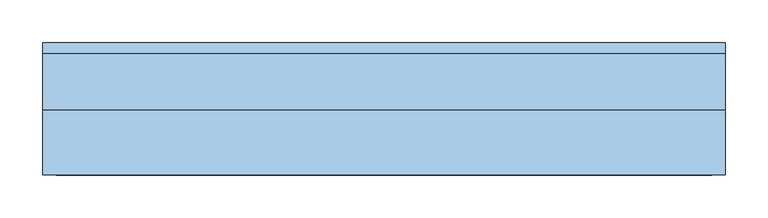
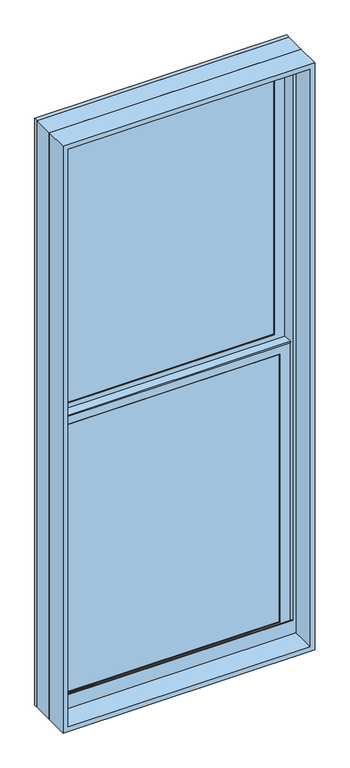
"""IFC4 building model written with IfcOpenShell, lengths in millimetres: window geometry, Window-Double_Hung-Marvin-Essential : ESDH2866."""

from ifc_helpers import new_model, si_unit, frame, origin, place, context, project, spatial, polyline, outline, extrude, faceted_brep, source, transform, mapped, element, save


def window_37e84bf3(model_context):
    return source(origin(), model_context, "Body", "SolidModel", [
        extrude(outline(polyline([(123.825, 20.6375), (123.825, 15.875), (104.775, 15.875), (104.775, 20.6375), (123.825, 20.6375)])), frame((0.0, 0.0, 527.05), z_axis=(0.0, 0.0, 1.0), x_axis=(1.0, 0.0, 0.0)), (0.0, 0.0, 1.0), 908.05),
        extrude(outline(polyline([(-104.775, 20.6375), (-104.775, 15.875), (-123.825, 15.875), (-123.825, 20.6375), (-104.775, 20.6375)])), frame((0.0, 0.0, 527.05), z_axis=(0.0, 0.0, 1.0), x_axis=(1.0, 0.0, 0.0)), (0.0, 0.0, 1.0), 908.05),
        extrude(outline(polyline([(342.9, 20.6375), (342.9, 15.875), (-342.9, 15.875), (-342.9, 20.6375), (342.9, 20.6375)])), frame((0.0, 0.0, 971.55), z_axis=(0.0, 0.0, 1.0), x_axis=(1.0, 0.0, 0.0)), (0.0, 0.0, 1.0), 19.05),
        extrude(outline(polyline([(-123.825, 46.83125), (-123.825, 51.59375), (-104.775, 51.59375), (-104.775, 46.83125), (-123.825, 46.83125)])), frame((0.0, 0.0, 1473.2), z_axis=(0.0, 0.0, 1.0), x_axis=(1.0, 0.0, 0.0)), (0.0, 0.0, 1.0), 908.05),
        extrude(outline(polyline([(104.775, 46.83125), (104.775, 51.59375), (123.825, 51.59375), (123.825, 46.83125), (104.775, 46.83125)])), frame((0.0, 0.0, 1473.2), z_axis=(0.0, 0.0, 1.0), x_axis=(1.0, 0.0, 0.0)), (0.0, 0.0, 1.0), 908.05),
        extrude(outline(polyline([(-342.9, 46.83125), (-342.9, 51.59375), (342.9, 51.59375), (342.9, 46.83125), (-342.9, 46.83125)])), frame((0.0, 0.0, 1917.7), z_axis=(0.0, 0.0, 1.0), x_axis=(1.0, 0.0, 0.0)), (0.0, 0.0, 1.0), 19.05),
        extrude(outline(polyline([(123.825, 20.6375), (104.775, 20.6375), (104.775, 25.4), (123.825, 25.4), (123.825, 20.6375)])), frame((0.0, 0.0, 527.05), z_axis=(0.0, 0.0, 1.0), x_axis=(1.0, 0.0, 0.0)), (0.0, 0.0, 1.0), 908.05),
        extrude(outline(polyline([(-104.775, 20.6375), (-123.825, 20.6375), (-123.825, 25.4), (-104.775, 25.4), (-104.775, 20.6375)])), frame((0.0, 0.0, 527.05), z_axis=(0.0, 0.0, 1.0), x_axis=(1.0, 0.0, 0.0)), (0.0, 0.0, 1.0), 908.05),
        extrude(outline(polyline([(342.9, 20.6375), (-342.9, 20.6375), (-342.9, 25.4), (342.9, 25.4), (342.9, 20.6375)])), frame((0.0, 0.0, 971.55), z_axis=(0.0, 0.0, 1.0), x_axis=(1.0, 0.0, 0.0)), (0.0, 0.0, 1.0), 19.05),
        extrude(outline(polyline([(-123.825, 56.35625), (-104.775, 56.35625), (-104.775, 51.59375), (-123.825, 51.59375), (-123.825, 56.35625)])), frame((0.0, 0.0, 1473.2), z_axis=(0.0, 0.0, 1.0), x_axis=(1.0, 0.0, 0.0)), (0.0, 0.0, 1.0), 908.05),
        extrude(outline(polyline([(104.775, 56.35625), (123.825, 56.35625), (123.825, 51.59375), (104.775, 51.59375), (104.775, 56.35625)])), frame((0.0, 0.0, 1473.2), z_axis=(0.0, 0.0, 1.0), x_axis=(1.0, 0.0, 0.0)), (0.0, 0.0, 1.0), 908.05),
        extrude(outline(polyline([(-342.9, 56.35625), (342.9, 56.35625), (342.9, 51.59375), (-342.9, 51.59375), (-342.9, 56.35625)])), frame((0.0, 0.0, 1917.7), z_axis=(0.0, 0.0, 1.0), x_axis=(1.0, 0.0, 0.0)), (0.0, 0.0, 1.0), 19.05),
        faceted_brep([(-369.8875, 5.6780605, 1465.1351748), (-369.8875, 5.6780605, 1460.5), (369.8875, 5.6780605, 1460.5), (369.8875, 5.6780605, 1465.1351748), (-369.8875, 34.8118605, 1465.1351748), (369.8875, 34.8118605, 1465.1351748), (369.8875, 34.8118605, 1460.5), (-369.8875, 34.8118605, 1460.5), (-369.8875, 30.1625, 1460.5), (-369.8875, 30.1625, 500.0625), (-369.8875, 8.9241104, 500.0625), (-369.8875, 8.9241104, 1460.5), (369.8875, 8.9241104, 1460.5), (369.8875, 30.1625, 1460.5), (369.8875, 8.9241104, 500.0625), (369.8875, 30.1625, 500.0625), (-354.0034752, 11.90625, 1446.2034752), (-354.0034752, 30.1625, 1446.2034752), (354.0034752, 30.1625, 1446.2034752), (354.0034752, 11.90625, 1446.2034752), (-337.34375, 10.4662439, 1429.54375), (-337.34375, 11.90625, 1429.54375), (337.34375, 11.90625, 1429.54375), (337.34375, 10.4662439, 1429.54375), (338.8858834, 8.9241104, 1431.0858834), (-338.8858834, 8.9241104, 1431.0858834), (354.0034752, 30.1625, 515.9465248), (354.0034752, 11.90625, 515.9465248), (337.34375, 11.90625, 532.60625), (337.34375, 10.4662439, 532.60625), (338.8858834, 8.9241104, 531.0641166), (-354.0034752, 30.1625, 515.9465248), (-354.0034752, 11.90625, 515.9465248), (-337.34375, 11.90625, 532.60625), (-337.34375, 10.4662439, 532.60625), (-338.8858834, 8.9241104, 531.0641166)], [[[0, 1, 2, 3]], [[4, 5, 6, 7]], [[1, 0, 4, 7, 8, 9, 10, 11]], [[2, 1, 11, 12]], [[7, 6, 13, 8]], [[3, 2, 12, 14, 15, 13, 6, 5]], [[0, 3, 5, 4]], [[16, 17, 18, 19]], [[20, 21, 22, 23]], [[20, 23, 24, 25]], [[19, 18, 26, 27]], [[23, 22, 28, 29]], [[24, 23, 29, 30]], [[27, 26, 31, 32]], [[29, 28, 33, 34]], [[30, 29, 34, 35]], [[15, 14, 10, 9]], [[15, 9, 8, 13], [18, 17, 31, 26]], [[17, 16, 32, 31]], [[16, 19, 27, 32], [22, 21, 33, 28]], [[21, 20, 34, 33]], [[20, 25, 35, 34]], [[10, 14, 12, 11], [25, 24, 30, 35]]]),
        extrude(outline(polyline([(38.5955581, 1446.2125), (33.5778968, 1446.2125), (33.5778968, 1447.8), (39.9405976, 1447.8), (39.9405976, 1446.2125), (61.515625, 1446.2125), (47.6307501, 1442.8975159), (38.5955581, 1442.8975159), (38.5955581, 1446.2125)])), frame((-369.8875, 0.0, 0.0), z_axis=(1.0, 0.0, 0.0), x_axis=(0.0, 1.0, 0.0)), (0.0, 0.0, 1.0), 739.775),
        faceted_brep([(400.05, 0.0, 469.9), (400.05, 0.0, 2438.4), (-400.05, 0.0, 2438.4), (-400.05, 0.0, 469.9), (373.85625, 0.0, 531.01875), (-373.85625, 0.0, 531.01875), (-373.85625, 0.0, 2412.20625), (373.85625, 0.0, 2412.20625), (373.85625, 3.96875, 469.9), (-373.85625, 3.96875, 469.9), (-373.85625, 3.96875, 531.01875), (373.85625, 3.96875, 531.01875), (-400.05, 65.6828125, 469.9), (-373.85625, 65.6828125, 469.9), (373.85625, 65.6828125, 469.9), (400.05, 65.6828125, 469.9), (-400.05, 65.6828125, 2438.4), (400.05, 65.6828125, 2438.4), (373.85625, 65.6828125, 2412.20625), (-373.85625, 65.6828125, 2412.20625)], [[[0, 1, 2, 3], [4, 5, 6, 7]], [[8, 9, 10, 11]], [[5, 4, 11, 10]], [[0, 3, 12, 13, 9, 8, 14, 15]], [[13, 12, 16, 17, 15, 14, 18, 19]], [[13, 19, 6, 5, 10, 9]], [[7, 6, 19, 18]], [[18, 14, 8, 11, 4, 7]], [[1, 0, 15, 17]], [[2, 1, 17, 16]], [[3, 2, 16, 12]]]),
        faceted_brep([(373.85625, 30.1625, 1454.15), (372.26875, 30.1625, 1454.15), (372.26875, 30.1625, 494.2544613), (373.85625, 30.1625, 494.2544613), (-372.26875, 30.1625, 1454.15), (-373.85625, 30.1625, 1454.15), (-373.85625, 30.1625, 494.2544613), (-372.26875, 30.1625, 494.2544613), (372.26875, 63.5, 1454.15), (373.85625, 63.5, 1454.15), (373.85625, 63.5, 487.7743077), (372.26875, 63.5, 487.7743077), (-373.85625, 63.5, 1454.15), (-372.26875, 63.5, 1454.15), (-372.26875, 63.5, 487.7743077), (-373.85625, 63.5, 487.7743077), (385.1108932, 3.96875, 499.3460105), (385.1108932, 3.96875, 469.9), (385.1108932, 65.6828125, 469.9), (385.1108932, 65.6828125, 487.350012), (-385.1108932, 3.96875, 469.9), (-385.1108932, 3.96875, 499.3460105), (-385.1108932, 65.6828125, 487.350012), (-385.1108932, 65.6828125, 469.9), (385.1108932, 78.58125, 484.8428097), (-385.1108932, 78.58125, 484.8428097), (-383.0971252, 68.2348864, 486.8539391), (-365.13135, 68.2348864, 486.8539391), (-365.13135, 65.6828125, 487.350012), (365.13135, 65.6828125, 487.350012), (365.13135, 68.2348864, 486.8539391), (383.0971252, 68.2348864, 486.8539391), (-400.05, 65.6828125, 469.9), (-400.05, 78.5948249, 469.9), (400.05, 78.5948249, 469.9), (400.05, 65.6828125, 469.9), (-400.05, 78.58125, 2438.4), (400.05, 78.58125, 2438.4), (385.1108932, 78.58125, 2423.4608932), (-385.1108932, 78.58125, 2423.4608932), (-400.05, 65.6828125, 2438.4), (-383.0971252, 68.2348864, 2421.4471252), (383.0971252, 68.2348864, 2421.4471252), (365.13135, 68.2348864, 2403.48135), (-365.13135, 68.2348864, 2403.48135), (-365.13135, 65.6828125, 2403.48135), (365.13135, 65.6828125, 2403.48135), (400.05, 65.6828125, 2438.4)], [[[0, 1, 2, 3]], [[4, 5, 6, 7]], [[8, 9, 10, 11]], [[12, 13, 14, 15]], [[1, 8, 11, 2]], [[9, 0, 3, 10]], [[1, 0, 9, 8]], [[5, 4, 13, 12]], [[5, 12, 15, 6]], [[13, 4, 7, 14]], [[16, 17, 18, 19]], [[20, 21, 22, 23]], [[24, 25, 26, 27, 28, 22, 21, 16, 19, 29, 30, 31], [3, 2, 11, 10], [7, 6, 15, 14]], [[17, 16, 21, 20]], [[17, 20, 23, 32, 33, 34, 35, 18]], [[34, 33, 36, 37], [25, 24, 38, 39]], [[33, 32, 40, 36]], [[39, 41, 26, 25]], [[41, 42, 31, 30, 43, 44, 27, 26]], [[44, 45, 28, 27]], [[40, 32, 23, 22, 28, 45, 46, 29, 19, 18, 35, 47]], [[36, 40, 47, 37]], [[39, 38, 42, 41]], [[44, 43, 46, 45]], [[34, 37, 47, 35]], [[42, 38, 24, 31]], [[46, 43, 30, 29]]]),
        extrude(outline(polyline([(350.04375, 11.90625), (-350.04375, 11.90625), (-350.04375, 15.08125), (350.04375, 15.08125), (350.04375, 11.90625)])), frame((0.0, 0.0, 519.90625), z_axis=(0.0, 0.0, 1.0), x_axis=(1.0, 0.0, 0.0)), (0.0, 0.0, 1.0), 922.3375),
        extrude(outline(polyline([(350.04375, 42.8625), (-350.04375, 42.8625), (-350.04375, 46.0375), (350.04375, 46.0375), (350.04375, 42.8625)])), frame((0.0, 0.0, 1466.05625), z_axis=(0.0, 0.0, 1.0), x_axis=(1.0, 0.0, 0.0)), (0.0, 0.0, 1.0), 922.3375),
        faceted_brep([(-337.34375, 31.194477, 1429.54375), (-338.8858834, 32.7366104, 1431.0858834), (338.8858834, 32.7366104, 1431.0858834), (337.34375, 31.194477, 1429.54375), (-337.34375, 30.1625, 1429.54375), (337.34375, 30.1625, 1429.54375), (-369.8875, 32.7366104, 1462.0875), (-369.8875, 30.1625, 1462.0875), (369.8875, 30.1625, 1462.0875), (369.8875, 32.7366104, 1462.0875), (338.8858834, 32.7366104, 531.0641166), (337.34375, 31.194477, 532.60625), (337.34375, 30.1625, 532.60625), (369.8875, 30.1625, 500.0625), (369.8875, 32.7366104, 500.0625), (-338.8858834, 32.7366104, 531.0641166), (-337.34375, 31.194477, 532.60625), (-337.34375, 30.1625, 532.60625), (-369.8875, 30.1625, 500.0625), (-369.8875, 32.7366104, 500.0625)], [[[0, 1, 2, 3]], [[4, 0, 3, 5]], [[6, 7, 8, 9]], [[3, 2, 10, 11]], [[5, 3, 11, 12]], [[9, 8, 13, 14]], [[11, 10, 15, 16]], [[12, 11, 16, 17]], [[14, 13, 18, 19]], [[9, 14, 19, 6], [1, 15, 10, 2]], [[16, 15, 1, 0]], [[17, 16, 0, 4]], [[7, 18, 13, 8], [5, 12, 17, 4]], [[19, 18, 7, 6]]]),
        faceted_brep([(-354.0034752, 42.8625, 2392.3534752), (-354.0034752, 61.11875, 2392.3534752), (354.0034752, 61.11875, 2392.3534752), (354.0034752, 42.8625, 2392.3534752), (-337.34375, 41.4224939, 2375.69375), (-337.34375, 42.8625, 2375.69375), (337.34375, 42.8625, 2375.69375), (337.34375, 41.4224939, 2375.69375), (-338.8858834, 39.8803604, 2377.2358834), (338.8858834, 39.8803604, 2377.2358834), (-369.8875, 61.11875, 2408.2375), (-369.8875, 39.8803604, 2408.2375), (369.8875, 39.8803604, 2408.2375), (369.8875, 61.11875, 2408.2375), (354.0034752, 61.11875, 1462.0965248), (354.0034752, 42.8625, 1462.0965248), (337.34375, 42.8625, 1478.75625), (337.34375, 41.4224939, 1478.75625), (338.8858834, 39.8803604, 1477.2141166), (369.8875, 39.8803604, 1446.2125), (369.8875, 61.11875, 1446.2125), (-354.0034752, 61.11875, 1462.0965248), (-354.0034752, 42.8625, 1462.0965248), (-337.34375, 42.8625, 1478.75625), (-337.34375, 41.4224939, 1478.75625), (-338.8858834, 39.8803604, 1477.2141166), (-369.8875, 39.8803604, 1446.2125), (-369.8875, 61.11875, 1446.2125)], [[[0, 1, 2, 3]], [[4, 5, 6, 7]], [[8, 4, 7, 9]], [[10, 11, 12, 13]], [[3, 2, 14, 15]], [[7, 6, 16, 17]], [[9, 7, 17, 18]], [[13, 12, 19, 20]], [[15, 14, 21, 22]], [[17, 16, 23, 24]], [[18, 17, 24, 25]], [[20, 19, 26, 27]], [[13, 20, 27, 10], [1, 21, 14, 2]], [[22, 21, 1, 0]], [[3, 15, 22, 0], [5, 23, 16, 6]], [[24, 23, 5, 4]], [[25, 24, 4, 8]], [[11, 26, 19, 12], [9, 18, 25, 8]], [[27, 26, 11, 10]]]),
        faceted_brep([(-369.8875, 61.11875, 1446.2125), (-369.8875, 63.6928604, 1446.2125), (369.8875, 63.6928604, 1446.2125), (369.8875, 61.11875, 1446.2125), (-337.34375, 62.150727, 1478.75625), (-337.34375, 61.11875, 1478.75625), (337.34375, 61.11875, 1478.75625), (337.34375, 62.150727, 1478.75625), (-338.8858834, 63.6928604, 1477.2141166), (338.8858834, 63.6928604, 1477.2141166), (369.8875, 63.6928604, 2408.2375), (369.8875, 61.11875, 2408.2375), (337.34375, 61.11875, 2375.69375), (337.34375, 62.150727, 2375.69375), (338.8858834, 63.6928604, 2377.2358834), (-369.8875, 63.6928604, 2408.2375), (-369.8875, 61.11875, 2408.2375), (-337.34375, 61.11875, 2375.69375), (-337.34375, 62.150727, 2375.69375), (-338.8858834, 63.6928604, 2377.2358834)], [[[0, 1, 2, 3]], [[4, 5, 6, 7]], [[8, 4, 7, 9]], [[3, 2, 10, 11]], [[7, 6, 12, 13]], [[9, 7, 13, 14]], [[11, 10, 15, 16]], [[13, 12, 17, 18]], [[14, 13, 18, 19]], [[16, 15, 1, 0]], [[3, 11, 16, 0], [5, 17, 12, 6]], [[18, 17, 5, 4]], [[19, 18, 4, 8]], [[1, 15, 10, 2], [9, 14, 19, 8]]]),
        extrude(outline(polyline([(350.04375, 26.19375), (-350.04375, 26.19375), (-350.04375, 30.1625), (350.04375, 30.1625), (350.04375, 26.19375)])), frame((0.0, 0.0, 519.90625), z_axis=(0.0, 0.0, 1.0), x_axis=(1.0, 0.0, 0.0)), (0.0, 0.0, 1.0), 922.3375),
        extrude(outline(polyline([(350.04375, 57.15), (-350.04375, 57.15), (-350.04375, 61.11875), (350.04375, 61.11875), (350.04375, 57.15)])), frame((0.0, 0.0, 1466.05625), z_axis=(0.0, 0.0, 1.0), x_axis=(1.0, 0.0, 0.0)), (0.0, 0.0, 1.0), 922.3375),
        extrude(outline(polyline([(2438.4, 400.05), (2438.4, -400.05), (469.9, -400.05), (469.9, 400.05), (2438.4, 400.05)]), holes=[polyline([(2422.525, 384.175), (485.775, 384.175), (485.775, -384.175), (2422.525, -384.175), (2422.525, 384.175)])]), frame((0.0, -76.2, 0.0), z_axis=(0.0, 1.0, 0.0), x_axis=(0.0, 0.0, 1.0)), (0.0, 0.0, 1.0), 75.40625),
    ])


if __name__ == "__main__":
    model = new_model("IFC4")
    model_context = context("Model", 3, world=origin())
    ifc_project = project(units=[si_unit("LENGTHUNIT", "METRE", prefix="MILLI")], contexts=[model_context])
    site = spatial("IfcSite", under=ifc_project)
    building = spatial("IfcBuilding", under=site)
    placement = place(None, origin())
    window_shape = window_37e84bf3(model_context)
    element("IfcWindow", 1, ObjectType="Window-Double_Hung-Marvin-Essential : ESDH2866", at=placement, inside=building, context=model_context, shape_type="MappedRepresentation", body=[
        mapped(window_shape, transform((0.0, 0.0, 0.0), x_axis=(1.0, 0.0, 0.0), y_axis=(0.0, 1.0, 0.0), z_axis=(0.0, 0.0, 1.0))),
    ])
    save(model, "model.ifc")

# Revit data of these elements
# Type "Window-Double_Hung-Marvin-Essential : ESDH2866"
#   Type Mark = "85"
#   Window Type = "Essential Double Hung"
#   Product data url = "https://bimobject.com/marvin-windows-and-doors/product/marvin-dhwau"
#   Product Guid = "c4a96547-874c-4385-91dc-a058adc19d98"
#   Frame = "All Ultrex"
#   Egress Window = "Yes"
#   URL = "www.marvin.com"
#   Model = "ESDH2866"
#   Manufacturer = "Marvin Windows and Doors"
#   Label Egress = "EGRESS WDW"
#   Glass Type = "IG Low E II with Argon"
#   Design Pressure = "DP50"
#   Description = "3278 DBHG"
#   Analytic Construction = "<None>"
#   Prairie Corner Width = 0' - 4"
#   Prairie Corner Height = 0' - 4"
#   Egress Width = 2' - 4 9/16"
#   Egress Height = 2' - 10 27/128"
#   Rough Width = 2' - 8"
#   Rough Height = 6' - 6"
#   Nominal Width = 2' - 8"
#   Nominal Height = 6' - 6"
#   Inset to Installation Flange [instance default] = 0' - 1"
#   Height = 6' - 5 1/2"
#   Egress Area = 6.78576 SF
#   Default Head Height = 8' - 0"
#   Width = 2' - 7 1/2"
#   Daylight Area = 13.0276 SF
#   DLO Width = 2' - 2 9/16"
#   DLO Height = 2' - 11 5/16"
#   Muntins Top Sash = yes
#   Lites Wide Top Sash = 3
#   Lites Wide Bottom Sash = 3
#   Lites High Top Sash = 2
#   Lites High Bottom Sash = 2
#   Lite Cut Prairie 9 = no
#   Lite Cut HV Grid = yes
#   Muntins Bottom Sash = yes
#   Label Visibility = no
#   Jamb Extension Visibility = yes
#   Edition number = 1
#   Interior Material = Ultrex-Marvin-Stonewhite
#   Glazing Material = Glass-Marvin-IG Low E II with Argon
#   Cladding Material = Ultrex-Marvin-Pebblegray
#   Wall Closure = (empty or 0)
#   Assembly Code = ""
# Element 1 (IfcWindow, "Window-Double_Hung-Marvin-Essential : ESDH2866")
#   Materials on its faces: "Ultrex-Marvin-Pebblegray", "Ultrex-Marvin-Stonewhite", "Glass-Marvin-IG Low E II with Argon"
# Materials
#   "Ultrex-Marvin-Stonewhite": class "Paint", colour RGB 250 251 245, transparency 0
#   "Glass-Marvin-IG Low E II with Argon": class "Glass", colour RGB 0 128 192, transparency 0.85
#   "Ultrex-Marvin-Pebblegray": class "Paint", colour RGB 189 185 173, transparency 0
